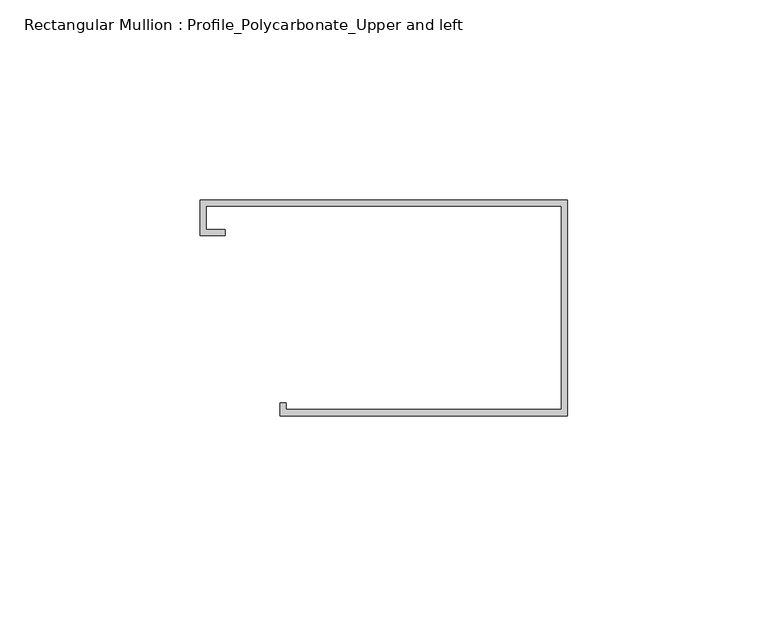
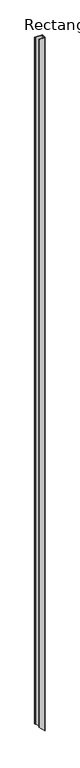
"""IFC4 building model written with IfcOpenShell, lengths in millimetres: member geometry, Rectangular Mullion : Profile_Polycarbonate_Upper and left."""

from ifc_helpers import new_model, si_unit, origin, place, context, project, spatial, faceted_brep, source, transform, mapped, element, save


def rectangular_mullion_profile_polycarbonate_upper_and_left_3fd8a9ea(model_context):
    return source(origin(), model_context, "Body", "Brep", [
        faceted_brep([(0.0, 28.984575, 0.0), (-91.9988, 28.984575, 0.0), (-91.9988, 19.992975, 0.0), (-85.6488, 19.992975, 0.0), (-85.6488, 21.580475, 0.0), (-90.4113, 21.580475, 0.0), (-90.4113, 27.397075, 0.0), (-1.5875, 27.397075, 0.0), (-1.5875, -23.428325, 0.0), (-70.3961, -23.428325, 0.0), (-70.3961, -21.840825, 0.0), (-71.9836, -21.840825, 0.0), (-71.9836, -25.015825, 0.0), (0.0, -25.015825, 0.0), (0.0, 28.984575, -8756.2051756), (-91.9988, 28.984575, -8667.9598335), (-91.9988, 19.992975, -8667.9598335), (-85.6488, 19.992975, -8674.0507599), (-85.6488, 21.580475, -8674.0507599), (-90.4113, 21.580475, -8669.4825651), (-90.4113, 27.397075, -8669.4825651), (-1.5875, 27.397075, -8754.682444), (-1.5875, -23.428325, -8754.682444), (-70.3961, -23.428325, -8688.6811652), (-70.3961, -21.840825, -8688.6811652), (-71.9836, -21.840825, -8687.1584336), (-71.9836, -25.015825, -8687.1584336), (0.0, -25.015825, -8756.2051756)], [[[0, 1, 2, 3, 4, 5, 6, 7, 8, 9, 10, 11, 12, 13]], [[1, 0, 14, 15]], [[2, 1, 15, 16]], [[3, 2, 16, 17]], [[4, 3, 17, 18]], [[5, 4, 18, 19]], [[6, 5, 19, 20]], [[7, 6, 20, 21]], [[8, 7, 21, 22]], [[9, 8, 22, 23]], [[10, 9, 23, 24]], [[11, 10, 24, 25]], [[12, 11, 25, 26]], [[13, 12, 26, 27]], [[0, 13, 27, 14]], [[14, 27, 26, 25, 24, 23, 22, 21, 20, 19, 18, 17, 16, 15]]]),
    ])


if __name__ == "__main__":
    model = new_model("IFC4")
    model_context = context("Model", 3, world=origin())
    ifc_project = project(units=[si_unit("LENGTHUNIT", "METRE", prefix="MILLI")], contexts=[model_context])
    site = spatial("IfcSite", under=ifc_project)
    building = spatial("IfcBuilding", under=site)
    placement = place(None, origin())
    rectangular_mullion_profile_polycarbonate_upper_and_left_shape = rectangular_mullion_profile_polycarbonate_upper_and_left_3fd8a9ea(model_context)
    element("IfcMember", 1, ObjectType="Rectangular Mullion : Profile_Polycarbonate_Upper and left", at=placement, inside=building, context=model_context, shape_type="MappedRepresentation", body=[
        mapped(rectangular_mullion_profile_polycarbonate_upper_and_left_shape, transform((0.0, 0.0, 0.0), x_axis=(1.0, 0.0, 0.0), y_axis=(0.0, 1.0, 0.0), z_axis=(0.0, 0.0, 1.0))),
    ])
    save(model, "model.ifc")

# Revit data of these elements
# Type "Rectangular Mullion : Profile_Polycarbonate_Upper and left"
#   built-in parameter 1007322 = 0.177167 (stored number, unit not read)
#   built-in parameter 1007321 = 0.00520833 (stored number, unit not read)
#   built-in parameter 1007320 = 0 (stored number, unit not read)
